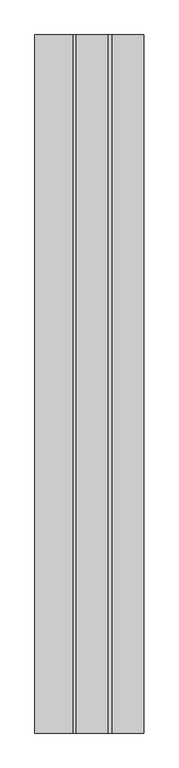
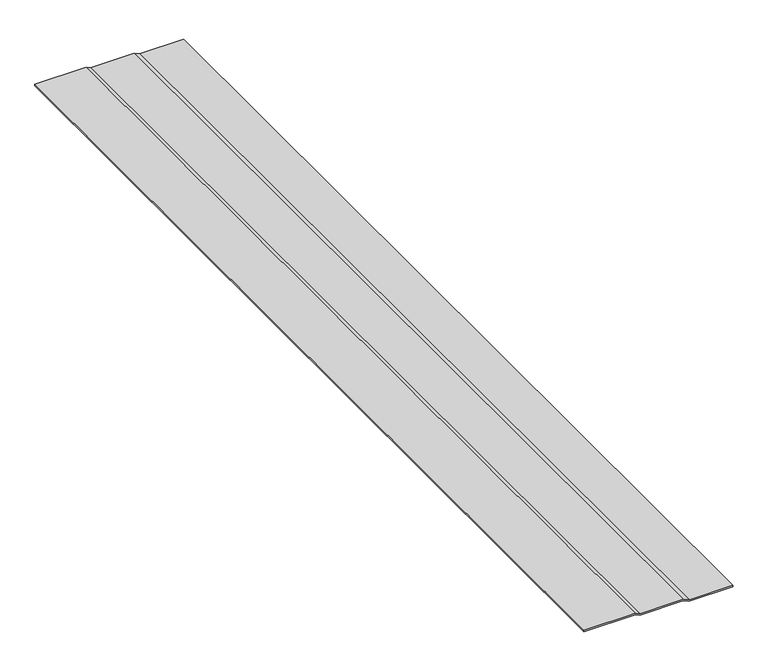
"""IFC4 building model written with IfcOpenShell, lengths in millimetres: proxy geometry, BITUMEN CAP SHEET2:BITUMEN CAP SHEET003:295613 : BITUMEN CAP SHEET2:BITUMEN CAP SHEET003:295613."""

from ifc_helpers import new_model, si_unit, frame, origin, place, context, project, spatial, polyline, outline, extrude, source, transform, mapped, element, save


def generic_models_0808d86b(model_context):
    return source(origin(), model_context, "Body", "SweptSolid", [
        extrude(outline(polyline([(40259.2002678, 2215.568251), (40259.2002678, 2307.7329126), (40262.3752679, 2307.7329126), (40262.3752679, 2216.213651), (40267.6612774, 2203.7488324), (40267.6612774, 2113.0650767), (40271.994072, 2103.3481752), (40271.994072, 1995.4616786), (40268.8188423, 1995.4616786), (40268.8188423, 2102.6728897), (40264.4862773, 2112.3892762), (40264.4862773, 2203.1034324), (40259.2002678, 2215.568251)])), frame((0.0, 1278.0825411, 0.0), z_axis=(0.0, 1.0, 0.0), x_axis=(0.0, 0.0, 1.0)), (0.0, 0.0, 1.0), 2000.25),
    ])


if __name__ == "__main__":
    model = new_model("IFC4")
    model_context = context("Model", 3, world=origin())
    ifc_project = project(units=[si_unit("LENGTHUNIT", "METRE", prefix="MILLI")], contexts=[model_context])
    site = spatial("IfcSite", under=ifc_project)
    building = spatial("IfcBuilding", under=site)
    placement = place(None, origin())
    generic_models_shape = generic_models_0808d86b(model_context)
    element("IfcBuildingElementProxy", 1, Name="BITUMEN CAP SHEET2:BITUMEN CAP SHEET003:295613 : BITUMEN CAP SHEET2:BITUMEN CAP SHEET003:295613", ObjectType="BITUMEN CAP SHEET2:BITUMEN CAP SHEET003:295613 : BITUMEN CAP SHEET2:BITUMEN CAP SHEET003:295613", at=placement, inside=building, context=model_context, shape_type="MappedRepresentation", body=[
        mapped(generic_models_shape, transform((0.0, 0.0, 0.0), x_axis=(1.0, 0.0, 0.0), y_axis=(0.0, 1.0, 0.0), z_axis=(0.0, 0.0, 1.0))),
    ])
    save(model, "model.ifc")

# Revit data of these elements
# Type "BITUMEN CAP SHEET2:BITUMEN CAP SHEET003:295613 : BITUMEN CAP SHEET2:BITUMEN CAP SHEET003:295613"
#   NameOverride = "BITUMEN CAP SHEET2:BITUMEN CAP SHEET003:295613"
#   ObjectTypeOverride = "BITUMEN CAP SHEET2:BITUMEN CAP SHEET003"
#   Reference = "BITUMEN CAP SHEET003"
#   Category = "Generic Models"
#   Tag = "295613"
# Element 1 (IfcBuildingElementProxy, "BITUMEN CAP SHEET2:BITUMEN CAP SHEET003:295613 : BITUMEN CAP SHEET2:BITUMEN CAP SHEET003:295613")
#   Materials on its faces: "MODIFIED BITUMEN GRANULE SURFACED CAP SHEET"
# Materials
#   "MODIFIED BITUMEN GRANULE SURFACED CAP SHEET": class "Unassigned", colour RGB 85 85 127, transparency 0
